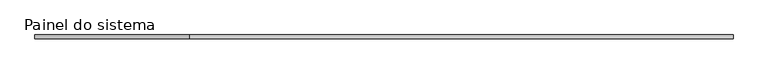
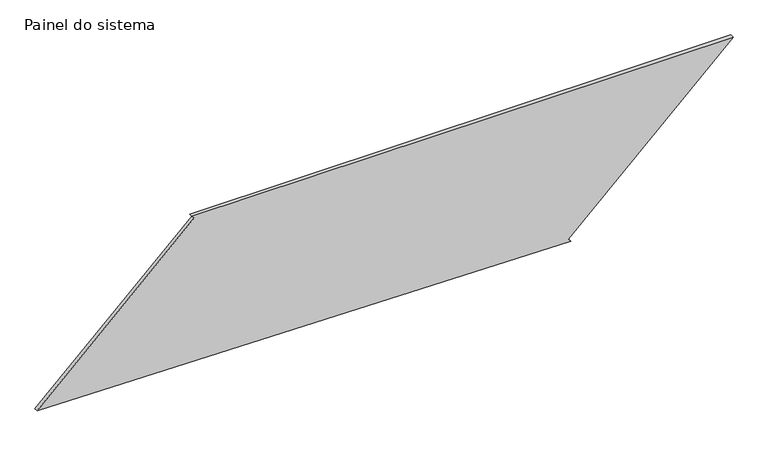
"""IFC4 building model written with IfcOpenShell, lengths in millimetres: plate geometry, Painel do sistema : Envidraçado."""

from ifc_helpers import new_model, si_unit, frame, origin, place, context, project, spatial, polyline, outline, extrude, source, transform, mapped, element, save


def painel_do_sistema_3a7d25bb(model_context):
    return source(origin(), model_context, "Body", "SweptSolid", [
        extrude(outline(polyline([(0.0, 1269.6890622), (18.146416, 1252.4929119), (1087.2313919, 2380.6559171), (1087.2313919, -1323.1220849), (1069.0849759, -1305.9259345), (50.6349184, -2380.6559171), (0.0, 1269.6890622)])), frame((0.0, 24.5, 0.0), z_axis=(0.0, 1.0, 0.0), x_axis=(0.0, 0.0, 1.0)), (0.0, 0.0, 1.0), 25.0),
    ])


if __name__ == "__main__":
    model = new_model("IFC4")
    model_context = context("Model", 3, world=origin())
    ifc_project = project(units=[si_unit("LENGTHUNIT", "METRE", prefix="MILLI")], contexts=[model_context])
    site = spatial("IfcSite", under=ifc_project)
    building = spatial("IfcBuilding", under=site)
    placement = place(None, origin())
    painel_do_sistema_shape = painel_do_sistema_3a7d25bb(model_context)
    element("IfcPlate", 1, ObjectType="Painel do sistema : Envidraçado", at=placement, inside=building, context=model_context, shape_type="MappedRepresentation", body=[
        mapped(painel_do_sistema_shape, transform((0.0, 0.0, 0.0), x_axis=(1.0, 0.0, 0.0), y_axis=(0.0, 1.0, 0.0), z_axis=(0.0, 0.0, 1.0))),
    ])
    save(model, "model.ifc")

# Revit data of these elements
# Type "Painel do sistema : Envidraçado"
#   Construction Type Id = "GSP4R"
#   Analytic Construction = "Vidraça única Pilkington 1/8 pol"
#   Visual Light Transmittance = 0.9
#   Solar Heat Gain Coefficient = 0.86
#   Heat Transfer Coefficient (U) = 6.7069 W/(m²·K)
# Element 1 (IfcPlate, "Painel do sistema : Envidraçado")
#   Materials on its faces: "Vidro"
# Materials
#   "Vidro": class "Vidro", colour RGB 0 128 192, transparency 0.9, Description = "Vidro de sílica", Cost = 0
